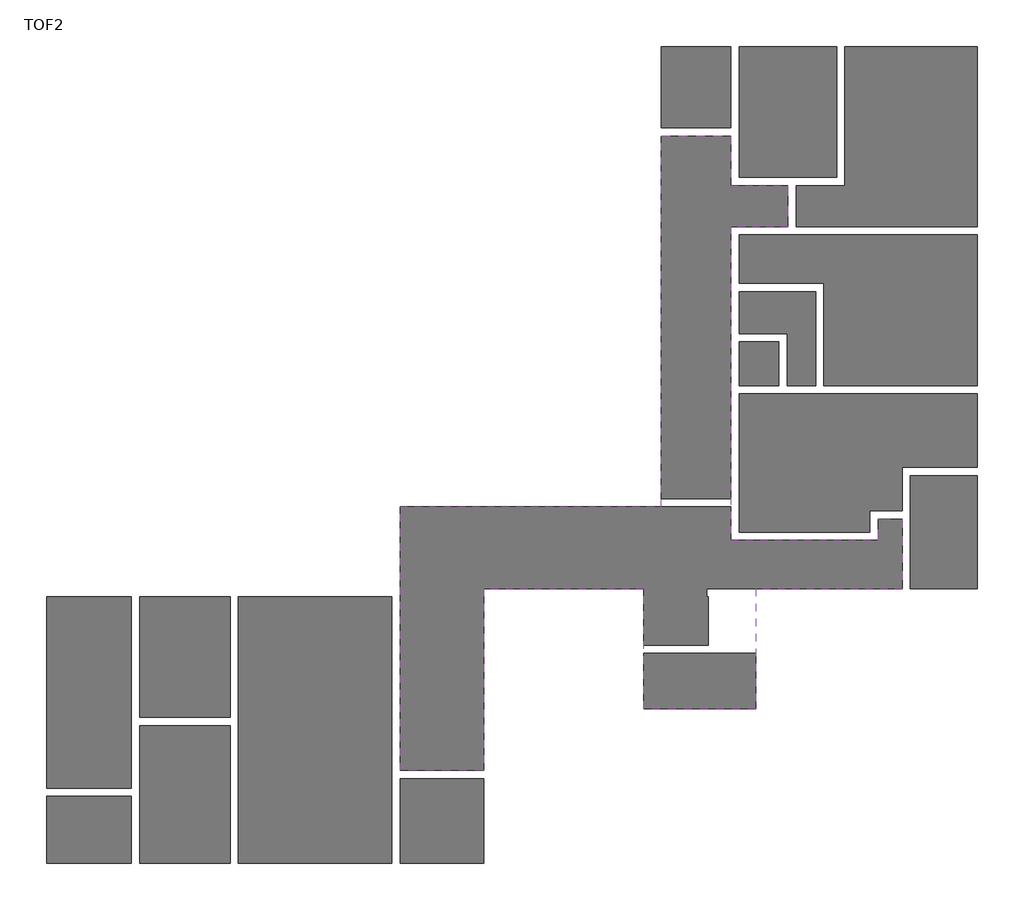
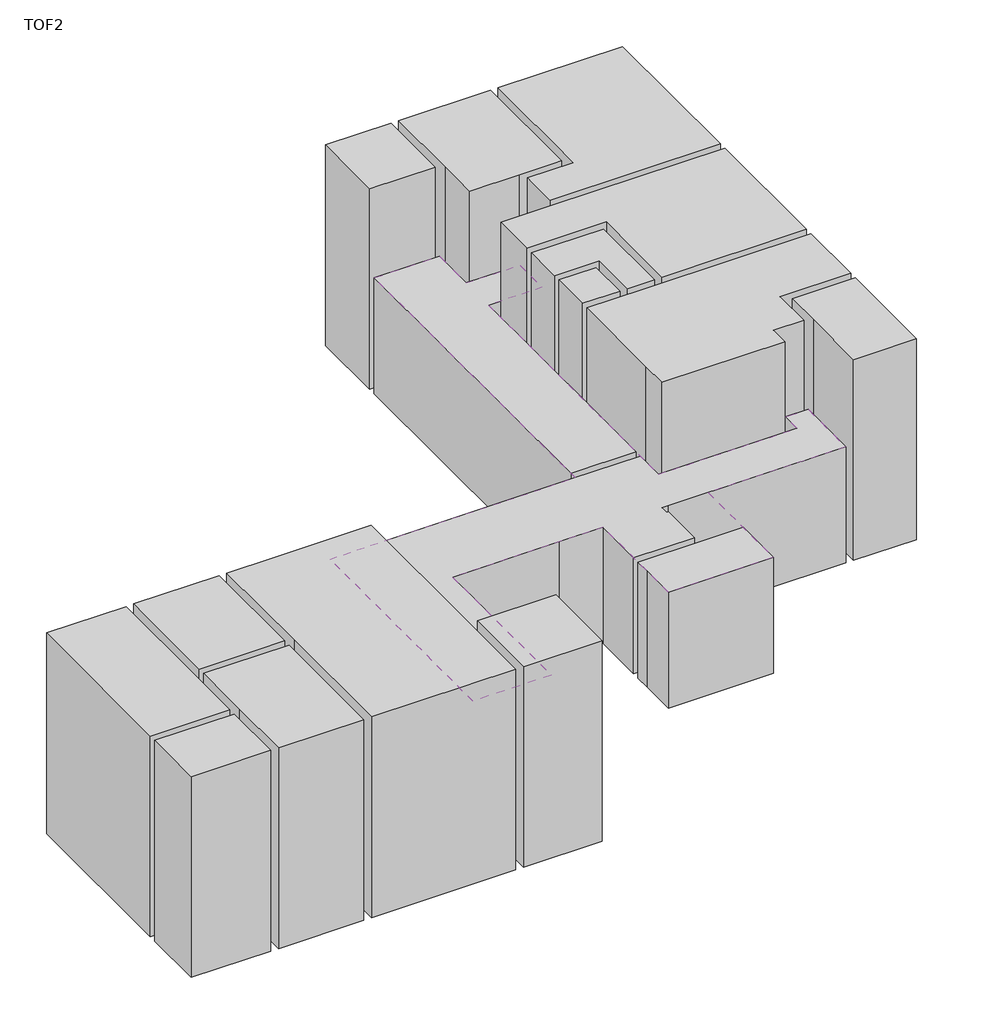
# One storey: 17 proxies, 1 covering.
"""IFC4 building model written with IfcOpenShell, lengths in millimetres."""

from ifc_helpers import new_model, si_unit, frame, origin, place, context, project, spatial, polyline, outline, extrude, element, save

model = new_model("IFC4")

# Units and contexts
model_context = context("Model", 3, world=origin())
ifc_project = project(units=[si_unit("LENGTHUNIT", "METRE", prefix="MILLI")], contexts=[model_context])

# Site, building, storey
site = spatial("IfcSite", under=ifc_project)
building = spatial("IfcBuilding", under=site)
storey = spatial("IfcBuildingStorey", under=building, Name="TOF2", Elevation=1150.0)

# Proxies
placement = place(None, origin())
element("IfcBuildingElementProxy", 1, Name="Generic Models", at=placement, inside=storey, context=model_context, shape_type="SweptSolid", body=[
    extrude(outline(polyline([(29058.7, 8299.5208589), (31624.7, 8299.5208589), (31624.7, 4880.5208589), (29058.7, 4880.5208589), (29058.7, 8299.5208589)])), frame((0.0, 0.0, 1150.0), z_axis=(0.0, 0.0, 1.0), x_axis=(1.0, 0.0, 0.0)), (0.0, 0.0, 1.0), 6399.0),
])
element("IfcBuildingElementProxy", 2, Name="Generic Models", at=placement, inside=storey, context=model_context, shape_type="SweptSolid", body=[
    extrude(outline(polyline([(31624.7, 746.5208589), (29058.7, 746.5208589), (29058.7, 2763.5208589), (29058.7, 4646.5208589), (31624.7, 4646.5208589), (31624.7, 746.5208589)])), frame((0.0, 0.0, 1150.0), z_axis=(0.0, 0.0, 1.0), x_axis=(1.0, 0.0, 0.0)), (0.0, 0.0, 1.0), 6399.0),
])
element("IfcBuildingElementProxy", 3, Name="Generic Models", at=placement, inside=storey, context=model_context, shape_type="SweptSolid", body=[
    extrude(outline(polyline([(26424.7, 8299.5208589), (28824.7, 8299.5208589), (28824.7, 4763.5208589), (28824.7, 2880.5208589), (26424.7, 2880.5208589), (26424.7, 8299.5208589)])), frame((0.0, 0.0, 1150.0), z_axis=(0.0, 0.0, 1.0), x_axis=(1.0, 0.0, 0.0)), (0.0, 0.0, 1.0), 6399.0),
])
element("IfcBuildingElementProxy", 4, Name="Generic Models", at=placement, inside=storey, context=model_context, shape_type="SweptSolid", body=[
    extrude(outline(polyline([(28824.7, 746.5208589), (26424.7, 746.5208589), (26424.7, 2646.5208589), (28824.7, 2646.5208589), (28824.7, 746.5208589)])), frame((0.0, 0.0, 1150.0), z_axis=(0.0, 0.0, 1.0), x_axis=(1.0, 0.0, 0.0)), (0.0, 0.0, 1.0), 6399.0),
])
element("IfcBuildingElementProxy", 5, Name="Generic Models", at=placement, inside=storey, context=model_context, shape_type="SweptSolid", body=[
    extrude(outline(polyline([(52794.7, 14049.5208589), (52794.7, 11967.5208589), (50660.7, 11967.5208589), (50660.7, 10733.5208589), (49743.7, 10733.5208589), (49743.7, 10133.5208589), (46041.7, 10133.5208589), (46041.7, 10966.5208589), (46041.7, 14049.5208589), (46824.7, 14049.5208589), (47924.7, 14049.5208589), (52794.7, 14049.5208589)])), frame((0.0, 0.0, 1150.0), z_axis=(0.0, 0.0, 1.0), x_axis=(1.0, 0.0, 0.0)), (0.0, 0.0, 1.0), 6399.0),
])
element("IfcBuildingElementProxy", 6, Name="Generic Models", at=placement, inside=storey, context=model_context, shape_type="SweptSolid", body=[
    extrude(outline(polyline([(52794.7, 18549.5208589), (52794.7, 14283.5208589), (48441.7, 14283.5208589), (48441.7, 17180.5208589), (46041.7, 17180.5208589), (46041.7, 18549.5208589), (47541.7, 18549.5208589), (52794.7, 18549.5208589)])), frame((0.0, 0.0, 1150.0), z_axis=(0.0, 0.0, 1.0), x_axis=(1.0, 0.0, 0.0)), (0.0, 0.0, 1.0), 6399.0),
])
element("IfcBuildingElementProxy", 7, Name="Generic Models", at=placement, inside=storey, context=model_context, shape_type="SweptSolid", body=[
    extrude(outline(polyline([(46041.7, 15754.2234045), (46041.7, 16946.5208589), (48207.7, 16946.5208589), (48207.7, 14283.5208589), (47401.7, 14283.5208589), (47401.7, 15754.2234045), (46041.7, 15754.2234045)])), frame((0.0, 0.0, 1150.0), z_axis=(0.0, 0.0, 1.0), x_axis=(1.0, 0.0, 0.0)), (0.0, 0.0, 1.0), 6399.0),
])
element("IfcBuildingElementProxy", 8, Name="Generic Models", at=placement, inside=storey, context=model_context, shape_type="SweptSolid", body=[
    extrude(outline(polyline([(46041.7, 14283.5208589), (46041.7, 15520.2234045), (47167.7, 15520.2234045), (47167.7, 14283.5208589), (46041.7, 14283.5208589)])), frame((0.0, 0.0, 1150.0), z_axis=(0.0, 0.0, 1.0), x_axis=(1.0, 0.0, 0.0)), (0.0, 0.0, 1.0), 6399.0),
])
element("IfcBuildingElementProxy", 9, Name="Generic Models", at=placement, inside=storey, context=model_context, shape_type="SweptSolid", body=[
    extrude(outline(polyline([(43841.7, 23886.5208589), (45807.7, 23886.5208589), (45807.7, 21586.5208589), (43841.7, 21586.5208589), (43841.7, 23886.5208589)])), frame((0.0, 0.0, 1150.0), z_axis=(0.0, 0.0, 1.0), x_axis=(1.0, 0.0, 0.0)), (0.0, 0.0, 1.0), 6399.0),
])
element("IfcBuildingElementProxy", 10, Name="Generic Models", at=placement, inside=storey, context=model_context, shape_type="SweptSolid", body=[
    extrude(outline(polyline([(46041.7, 23886.5208589), (48807.7, 23886.5208589), (48807.7, 20183.5208589), (47541.7, 20183.5208589), (46041.7, 20183.5208589), (46041.7, 21469.5208589), (46041.7, 23886.5208589)])), frame((0.0, 0.0, 1150.0), z_axis=(0.0, 0.0, 1.0), x_axis=(1.0, 0.0, 0.0)), (0.0, 0.0, 1.0), 6399.0),
])
element("IfcBuildingElementProxy", 11, Name="Generic Models", at=placement, inside=storey, context=model_context, shape_type="SweptSolid", body=[
    extrude(outline(polyline([(49041.7, 23886.5208589), (52794.7, 23886.5208589), (52794.7, 18783.5208589), (47658.7, 18783.5208589), (47658.7, 19949.5208589), (49041.7, 19949.5208589), (49041.7, 23886.5208589)])), frame((0.0, 0.0, 1150.0), z_axis=(0.0, 0.0, 1.0), x_axis=(1.0, 0.0, 0.0)), (0.0, 0.0, 1.0), 6399.0),
])
element("IfcBuildingElementProxy", 12, Name="Generic Models", at=placement, inside=storey, context=model_context, shape_type="SweptSolid", body=[
    extrude(outline(polyline([(52794.7, 11733.5208589), (52794.7, 8533.5208589), (50894.7, 8533.5208589), (50894.7, 10616.5208589), (50894.7, 11733.5208589), (52794.7, 11733.5208589)])), frame((0.0, 0.0, 1150.0), z_axis=(0.0, 0.0, 1.0), x_axis=(1.0, 0.0, 0.0)), (0.0, 0.0, 1.0), 6399.0),
])
element("IfcBuildingElementProxy", 13, Name="Generic Models", at=placement, inside=storey, context=model_context, shape_type="SweptSolid", body=[
    extrude(outline(polyline([(36207.7, 746.5208589), (31858.7, 746.5208589), (31858.7, 4763.5208589), (31858.7, 8299.5208589), (33274.7, 8299.5208589), (36207.7, 8299.5208589), (36207.7, 3263.5208589), (36207.7, 746.5208589)])), frame((0.0, 0.0, 1150.0), z_axis=(0.0, 0.0, 1.0), x_axis=(1.0, 0.0, 0.0)), (0.0, 0.0, 1.0), 6399.0),
])
element("IfcBuildingElementProxy", 14, Name="Generic Models", at=placement, inside=storey, context=model_context, shape_type="SweptSolid", body=[
    extrude(outline(polyline([(38807.7, 746.5208589), (36441.7, 746.5208589), (36441.7, 3146.5208589), (38807.7, 3146.5208589), (38807.7, 746.5208589)])), frame((0.0, 0.0, 1150.0), z_axis=(0.0, 0.0, 1.0), x_axis=(1.0, 0.0, 0.0)), (0.0, 0.0, 1.0), 6399.0),
])
element("IfcBuildingElementProxy", 15, Name="Generic Models", at=placement, inside=storey, context=model_context, shape_type="SweptSolid", body=[
    extrude(outline(polyline([(36441.7, 3380.5208589), (36441.7, 8416.5208589), (36441.7, 10849.5208589), (43724.7, 10849.5208589), (45807.7, 10849.5208589), (45807.7, 9899.5208589), (49977.7, 9899.5208589), (49977.7, 10499.5208589), (50660.7, 10499.5208589), (50660.7, 8533.5208589), (45292.8778017, 8533.5208589), (45124.7, 8533.5208589), (45124.7, 8299.5208589), (45175.8778017, 8299.5208589), (45175.8778017, 6933.5208589), (43341.7, 6933.5208589), (43341.7, 8533.5208589), (42007.7, 8533.5208589), (38807.7, 8533.5208589), (38807.7, 6963.5208589), (38807.7, 5013.5208589), (38807.7, 3380.5208589), (36441.7, 3380.5208589)])), frame((0.0, 0.0, 1150.0), z_axis=(0.0, 0.0, 1.0), x_axis=(1.0, 0.0, 0.0)), (0.0, 0.0, 1.0), 3700.0),
])
element("IfcBuildingElementProxy", 16, Name="Generic Models", at=placement, inside=storey, context=model_context, shape_type="SweptSolid", body=[
    extrude(outline(polyline([(46507.7, 6699.5208589), (46507.7, 5130.5208589), (43341.7, 5130.5208589), (43341.7, 6216.5208589), (43341.7, 6699.5208589), (45292.8778017, 6699.5208589), (46507.7, 6699.5208589)])), frame((0.0, 0.0, 1150.0), z_axis=(0.0, 0.0, 1.0), x_axis=(1.0, 0.0, 0.0)), (0.0, 0.0, 1.0), 3700.0),
])
element("IfcBuildingElementProxy", 17, Name="Generic Models", at=placement, inside=storey, context=model_context, shape_type="SweptSolid", body=[
    extrude(outline(polyline([(45807.7, 11083.5208589), (43841.7, 11083.5208589), (43841.7, 21352.5208589), (45807.7, 21352.5208589), (45807.7, 19949.5208589), (47424.7, 19949.5208589), (47424.7, 18783.5208589), (45807.7, 18783.5208589), (45807.7, 16283.5208589), (45807.7, 15183.5208589), (45807.7, 14166.5208589), (45807.7, 11083.5208589)])), frame((0.0, 0.0, 1150.0), z_axis=(0.0, 0.0, 1.0), x_axis=(1.0, 0.0, 0.0)), (0.0, 0.0, 1.0), 3700.0),
])

# Covering
element("IfcCovering", 18, ObjectType="CE741_Acoustic Tiled Ceiling System_600x600x9t_T_bar", at=placement, inside=storey, context=model_context, shape_type="SweptSolid", body=[
    extrude(outline(polyline([(46507.7, 8533.5208589), (46507.7, 5130.5208589), (43341.7, 5130.5208589), (43341.7, 8533.5208589), (38807.7, 8533.5208589), (38807.7, 3380.5208589), (36441.7, 3380.5208589), (36441.7, 10849.5208589), (43841.7, 10849.5208589), (43841.7, 21352.5208589), (45807.7, 21352.5208589), (45807.7, 19949.5208589), (47424.7, 19949.5208589), (47424.7, 18783.5208589), (45807.7, 18783.5208589), (45807.7, 9899.5208589), (49977.7, 9899.5208589), (49977.7, 10499.5208589), (50660.7, 10499.5208589), (50660.7, 8533.5208589), (46507.7, 8533.5208589)])), frame((0.0, 0.0, 4850.0), z_axis=(0.0, 0.0, 1.0), x_axis=(1.0, 0.0, 0.0)), (0.0, 0.0, 1.0), 9.0),
])

save(model, "model.ifc")

# Revit data of these elements
# Project information
#   Building Name = "SULFUR LOADING CONTROL BD"
#   Project Status = "Project Status"
#   Client Name = "현대엔지니어링"
#   Project Address = "서울시 종로구 율곡로 75(계동)"
#   Project Number = "-"
# Grids (mm)
#   "Y1": line (-3935.398, 24016.521) -> (58968.688, 24016.521)
#   "X1": line (-75.3, 29394.337) -> (-75.3, -4379.638)
#   "X2": line (5924.7, 29394.337) -> (5924.7, -4379.638)
#   "Y3": line (-3935.398, 8416.521) -> (58968.688, 8416.521)
#   "Y4": line (-3935.398, 616.521) -> (58968.688, 616.521)
#   "X3": line (11924.7, 29394.337) -> (11924.7, -4379.638)
#   "X4": line (17924.7, 29394.337) -> (17924.7, -4379.638)
#   "X5": line (26124.7, 29394.337) -> (26124.7, -4379.638)
#   "X6": line (31924.7, 29394.337) -> (31924.7, -4379.638)
#   "X7": line (38924.7, 29394.337) -> (38924.7, -4379.638)
#   "X8": line (45924.7, 29394.337) -> (45924.7, -4379.638)
#   "X9": line (52924.7, 29394.337) -> (52924.7, -4379.638)
#   "X15": line (43724.7, 27041.858) -> (43724.7, 9156.488)
#   "X16": line (36324.7, 27041.858) -> (36324.7, 9156.488)
#   "X17": line (34685.051, 10966.521) -> (55094.626, 10966.521)
#   "X18": line (34685.051, 18666.521) -> (55094.626, 18666.521)
#   "Y2": line (-3935.398, 12316.521) -> (58968.688, 12316.521)
# Type "CE741_Acoustic Tiled Ceiling System_600x600x9t_T_bar"
#   built-in parameter 1002203 = 1 (stored number, unit not read)
#   built-in parameter 1002202 = 1 (stored number, unit not read)
#   Layers, outside or top first: 9.000 mm no material (function 4)
# Elements 1, 2, 3, 4, 5, 6, 7, 8, 9, 10, 11, 12, 13, 14, 15, 16, 17 (IfcBuildingElementProxy)
#   Phase Created = New Construction
#   Materials on its faces: "Default"
# Element 18 (IfcCovering, "CE741_Acoustic Tiled Ceiling System_600x600x9t_T_bar")
#   Height Offset From Level = 3700.000 mm
#   Phase Created = New Construction
# Materials
#   "Default": class "Miscellaneous", colour RGB 80 80 80, transparency 0
# Room at (42616.2, 7496.521) mm, phase "New Construction", upper level "TOC", upper offset 6500.000 mm, lower offset -1000.000 mm
#   Comments = ""
#   Number = "127"
#   Name = "SHOWER ROOM"
#   Floor Finish Style Name = "Non-Slip Unglazed Ceramic Tile on Screed + Liquid Waterproofing"
#   Floor Finish Ref. = ""
#   Floor-Base Material = "Concrete Slab"
#   Floor Finish-1 = "Screed"
#   Floor Finish-2 = "Liquid Waterproofing"
#   Floor Finish-3 = "Ceramic Tile"
#   Floor Finish-4 = ""
#   Base Finish Style Name = "Epoxy Paint"
#   Base Finish Ref. = ""
#   Base-Base Material = "Concrete Wall\n/ Masonry Wall \n/ Dry Wall"
#   Base Finish-1 = ""
#   Base Finish-2 = ""
#   Base Finish-3 = "Epoxy Paint"
#   Base Finish-4 = ""
#   Wall Finish-1 = "Glazed Ceramic Tile on Cement Plaster"
#   Wall Finish-2 = "No Ceiling\nFull Height"
#   Wall Finish-3 = "Concrete Wall\n/ Masonry Wall"
#   Wall Finish-4 = "Plastering (Tile Workì í¬í¨)"
#   Ceiling Finish Style Name = "Suspended Moisture Resistant Tiled Ceiling (T-Bar)"
#   Ceiling Finish Ref. = "600x600\nT bar"
#   Ceiling-Base Material = "Concrete Slab"
#   Ceiling Finish-1 = ""
#   Ceiling Finish-2 = ""
#   Ceiling Finish-3 = "Moisture Resistant Tiled Ceiling System (T-Bar)"
#   Ceiling Finish-4 = ""
#   H_Room L = 1800.000 mm
#   H_Room W = 1200.000 mm
#   H_Room H or CH = 7300.000 mm
#   Floor Finish Style No = F31B
#   Base Finish Style No = B03
#   Wall Finish Style No = W32C
#   Ceiling Finish Style No = C96A
# Room at (42616.2, 5955.021) mm, phase "New Construction", upper level "TOC", upper offset 6500.000 mm, lower offset -1000.000 mm
#   Comments = ""
#   Number = "128"
#   Name = "EWH ROOM"
#   Floor Finish Style Name = "Non-Slip Unglazed Ceramic Tile on Screed"
#   Floor Finish Ref. = ""
#   Floor-Base Material = "Concrete Slab"
#   Floor Finish-1 = "Screed"
#   Floor Finish-2 = ""
#   Floor Finish-3 = "Ceramic Tile"
#   Floor Finish-4 = ""
#   Base Finish Style Name = "Epoxy Paint"
#   Base Finish Ref. = ""
#   Base-Base Material = "Concrete Wall\n/ Masonry Wall \n/ Dry Wall"
#   Base Finish-1 = ""
#   Base Finish-2 = ""
#   Base Finish-3 = "Epoxy Paint"
#   Base Finish-4 = ""
#   Wall Finish-1 = "Acrylic Emulsion Paint on Cement Plaster"
#   Wall Finish-2 = "T13 Plaster"
#   Wall Finish-3 = "Masonry Wall"
#   Wall Finish-4 = "Plastering"
#   Ceiling Finish Style Name = "Suspended Acoustic Tiled Ceiling (T-Bar)"
#   Ceiling Finish Ref. = "600x600\nT Bar"
#   Ceiling-Base Material = "Concrete Slab"
#   Ceiling Finish-1 = ""
#   Ceiling Finish-2 = ""
#   Ceiling Finish-3 = "Acoustic Tiled Ceiling System (T-Bar)"
#   Ceiling Finish-4 = ""
#   H_Room L = 1500.000 mm
#   H_Room W = 1200.000 mm
#   H_Room H or CH = 7300.000 mm
#   Floor Finish Style No = F31A
#   Base Finish Style No = B03
#   Wall Finish Style No = W01B
#   Ceiling Finish Style No = C95A
# Room at (30341.7, 6590.021) mm, phase "New Construction", upper level "TOC", upper offset 6500.000 mm, lower offset -1000.000 mm
#   Comments = ""
#   Number = "113"
#   Name = "STORE"
#   Floor Finish Style Name = "Vinyl Tile on Screed"
#   Floor Finish Ref. = ""
#   Floor-Base Material = "Concrete Slab"
#   Floor Finish-1 = "Screed"
#   Floor Finish-2 = ""
#   Floor Finish-3 = "Vinyl Tile"
#   Floor Finish-4 = ""
#   Base Finish Style Name = "Coved Vinyl Tile"
#   Base Finish Ref. = ""
#   Base-Base Material = "Concrete Wall\n/ Masonry Wall"
#   Base Finish-1 = ""
#   Base Finish-2 = ""
#   Base Finish-3 = "Vinyl Tile"
#   Base Finish-4 = ""
#   Wall Finish-1 = "Acrylic Emulsion Paint on Cement Plaster"
#   Wall Finish-2 = "T13 Plaster"
#   Wall Finish-3 = "Masonry Wall"
#   Wall Finish-4 = "Plastering"
#   Ceiling Finish Style Name = "Suspended Acoustic Tiled Ceiling (T-Bar)"
#   Ceiling Finish Ref. = "600x600\nT Bar"
#   Ceiling-Base Material = "Concrete Slab"
#   Ceiling Finish-1 = ""
#   Ceiling Finish-2 = ""
#   Ceiling Finish-3 = "Acoustic Tiled Ceiling System (T-Bar)"
#   Ceiling Finish-4 = ""
#   H_Room L = 3600.000 mm
#   H_Room W = 2700.000 mm
#   H_Room H or CH = 6300.000 mm
#   Floor Finish Style No = F34A
#   Base Finish Style No = B35A
#   Wall Finish Style No = W01B
#   Ceiling Finish Style No = C95A
# Room at (30341.7, 2647.521) mm, phase "New Construction", upper level "TOC", upper offset 6500.000 mm, lower offset -1000.000 mm
#   Comments = ""
#   Number = "115"
#   Name = "TELECOMS ROOM"
#   Floor Finish Style Name = "Vinyl Tile on Screed"
#   Floor Finish Ref. = ""
#   Floor-Base Material = "Concrete Slab"
#   Floor Finish-1 = "Screed"
#   Floor Finish-2 = ""
#   Floor Finish-3 = "Vinyl Tile"
#   Floor Finish-4 = ""
#   Base Finish Style Name = "Coved Vinyl Tile"
#   Base Finish Ref. = ""
#   Base-Base Material = "Concrete Wall\n/ Masonry Wall"
#   Base Finish-1 = ""
#   Base Finish-2 = ""
#   Base Finish-3 = "Vinyl Tile"
#   Base Finish-4 = ""
#   Wall Finish-1 = "2 Coats of Non-Conductive & Fire Retardant White Color Paint on Thk.13 Cement Plaster"
#   Wall Finish-2 = ""
#   Wall Finish-3 = ""
#   Wall Finish-4 = ""
#   Ceiling Finish Style Name = "Acrylic Emulsion Paint on Fair Faced Concrete"
#   Ceiling Finish Ref. = ""
#   Ceiling-Base Material = "Concrete Slab"
#   Ceiling Finish-1 = ""
#   Ceiling Finish-2 = ""
#   Ceiling Finish-3 = "Acrylic Emulsion Paint"
#   Ceiling Finish-4 = ""
#   H_Room L = 4200.000 mm
#   H_Room W = 2700.000 mm
#   H_Room H or CH = 6300.000 mm
#   Floor Finish Style No = F34A
#   Base Finish Style No = B35A
#   Wall Finish Style No = W11
#   Ceiling Finish Style No = C01
# Room at (27624.7, 5590.021) mm, phase "New Construction", upper level "TOC", upper offset 6500.000 mm, lower offset -1000.000 mm
#   Comments = ""
#   Number = "116"
#   Name = "CORRIDOR"
#   Floor Finish Style Name = "Vinyl Tile on Screed"
#   Floor Finish Ref. = ""
#   Floor-Base Material = "Concrete Slab"
#   Floor Finish-1 = "Screed"
#   Floor Finish-2 = ""
#   Floor Finish-3 = "Vinyl Tile"
#   Floor Finish-4 = ""
#   Base Finish Style Name = "Coved Vinyl Tile"
#   Base Finish Ref. = ""
#   Base-Base Material = "Concrete Wall\n/ Masonry Wall"
#   Base Finish-1 = ""
#   Base Finish-2 = ""
#   Base Finish-3 = "Vinyl Tile"
#   Base Finish-4 = ""
#   Wall Finish-1 = "Acrylic Emulsion Paint on Cement Plaster"
#   Wall Finish-2 = "T13 Plaster"
#   Wall Finish-3 = "Masonry Wall"
#   Wall Finish-4 = "Plastering"
#   Ceiling Finish Style Name = "Suspended Acoustic Tiled Ceiling (T-Bar)"
#   Ceiling Finish Ref. = "600x600\nT Bar"
#   Ceiling-Base Material = "Concrete Slab"
#   Ceiling Finish-1 = ""
#   Ceiling Finish-2 = ""
#   Ceiling Finish-3 = "Acoustic Tiled Ceiling System (T-Bar)"
#   Ceiling Finish-4 = ""
#   H_Room L = 5600.000 mm
#   H_Room W = 2600.000 mm
#   H_Room H or CH = 6300.000 mm
#   Floor Finish Style No = F34A
#   Base Finish Style No = B35A
#   Wall Finish Style No = W01B
#   Ceiling Finish Style No = C95A
# Room at (27624.7, 1647.521) mm, phase "New Construction", upper level "TOC", upper offset 6500.000 mm, lower offset -1000.000 mm
#   Comments = ""
#   Number = "117"
#   Name = "AIR LOCK"
#   Floor Finish Style Name = "Vinyl Tile on Screed + Matwell"
#   Base Finish Style Name = "Coved Vinyl Tile"
#   Base Finish Ref. = ""
#   Base-Base Material = "Concrete Wall\n/ Masonry Wall"
#   Base Finish-1 = ""
#   Base Finish-2 = ""
#   Base Finish-3 = "Vinyl Tile"
#   Base Finish-4 = ""
#   Wall Finish-1 = "Acrylic Emulsion Paint on Cement Plaster"
#   Wall Finish-2 = "T13 Plaster"
#   Wall Finish-3 = "Masonry Wall"
#   Wall Finish-4 = "Plastering"
#   Ceiling Finish Style Name = "Suspended Acoustic Tiled Ceiling (T-Bar)"
#   Ceiling Finish Ref. = "600x600\nT Bar"
#   Ceiling-Base Material = "Concrete Slab"
#   Ceiling Finish-1 = ""
#   Ceiling Finish-2 = ""
#   Ceiling Finish-3 = "Acoustic Tiled Ceiling System (T-Bar)"
#   Ceiling Finish-4 = ""
#   H_Room L = 2200.000 mm
#   H_Room W = 2600.000 mm
#   H_Room H or CH = 6300.000 mm
#   Floor Finish Style No = F34A-1
#   Base Finish Style No = B35A
#   Wall Finish Style No = W01B
#   Ceiling Finish Style No = C95A
# Room at (49467.2, 12091.521) mm, phase "New Construction", upper level "TOC", upper offset 6500.000 mm, lower offset -1000.000 mm
#   Comments = ""
#   Number = "111"
#   Name = "PRAYER ROOM"
#   Floor Finish Style Name = "Carpet Tile on Screed"
#   Floor Finish Ref. = ""
#   Floor-Base Material = "Concrete Slab"
#   Floor Finish-1 = "Screed"
#   Floor Finish-2 = ""
#   Floor Finish-3 = "Carpet Tile"
#   Floor Finish-4 = ""
#   Base Finish Style Name = "Coved Vinyl Tile"
#   Base Finish Ref. = ""
#   Base-Base Material = "Concrete Wall\n/ Masonry Wall"
#   Base Finish-1 = ""
#   Base Finish-2 = ""
#   Base Finish-3 = "Vinyl Tile"
#   Base Finish-4 = ""
#   Wall Finish-1 = "Acrylic Emulsion Paint on Cement Plaster"
#   Wall Finish-2 = "T13 Plaster"
#   Wall Finish-3 = "Masonry Wall"
#   Wall Finish-4 = "Plastering"
#   Ceiling Finish Style Name = "Suspended Acoustic Tiled Ceiling (T-Bar)"
#   Ceiling Finish Ref. = "600x600\nT Bar"
#   Ceiling-Base Material = "Concrete Slab"
#   Ceiling Finish-1 = ""
#   Ceiling Finish-2 = ""
#   Ceiling Finish-3 = "Acoustic Tiled Ceiling System (T-Bar)"
#   Ceiling Finish-4 = ""
#   H_Room L = 4100.000 mm
#   H_Room W = 7000.000 mm
#   H_Room H or CH = 6300.000 mm
#   Floor Finish Style No = F72
#   Base Finish Style No = B35A
#   Wall Finish Style No = W01B
#   Ceiling Finish Style No = C95A
# Room at (49867.2, 16696.521) mm, phase "New Construction", upper level "TOC", upper offset 6500.000 mm, lower offset -1000.000 mm
#   Comments = ""
#   Number = "108"
#   Name = "BREAK ROOM"
#   Floor Finish Style Name = "Vinyl Tile on Screed"
#   Floor Finish Ref. = ""
#   Floor-Base Material = "Concrete Slab"
#   Floor Finish-1 = "Screed"
#   Floor Finish-2 = ""
#   Floor Finish-3 = "Vinyl Tile"
#   Floor Finish-4 = ""
#   Base Finish Style Name = "Coved Vinyl Tile"
#   Base Finish Ref. = ""
#   Base-Base Material = "Concrete Wall\n/ Masonry Wall"
#   Base Finish-1 = ""
#   Base Finish-2 = ""
#   Base Finish-3 = "Vinyl Tile"
#   Base Finish-4 = ""
#   Wall Finish-1 = "Acrylic Emulsion Paint on Cement Plaster"
#   Wall Finish-2 = "T13 Plaster"
#   Wall Finish-3 = "Masonry Wall"
#   Wall Finish-4 = "Plastering"
#   Ceiling Finish Style Name = "Suspended Moisture Resistant Tiled Ceiling (T-Bar)"
#   Ceiling Finish Ref. = "600x600\nT bar"
#   Ceiling-Base Material = "Concrete Slab"
#   Ceiling Finish-1 = ""
#   Ceiling Finish-2 = ""
#   Ceiling Finish-3 = "Moisture Resistant Tiled Ceiling System (T-Bar)"
#   Ceiling Finish-4 = ""
#   H_Room L = 4500.000 mm
#   H_Room W = 7000.000 mm
#   H_Room H or CH = 6300.000 mm
#   Floor Finish Style No = F34A
#   Base Finish Style No = B35A
#   Wall Finish Style No = W01B
#   Ceiling Finish Style No = C96A
# Room at (47653.075, 16372.8) mm, phase "New Construction", upper level "TOC", upper offset 6500.000 mm, lower offset -1000.000 mm
#   Comments = ""
#   Number = "109"
#   Name = "JANITOR"
#   Floor Finish Style Name = "Non-Slip Unglazed Ceramic Tile on Screed + Liquid Waterproofing"
#   Floor Finish Ref. = ""
#   Floor-Base Material = "Concrete Slab"
#   Floor Finish-1 = "Screed"
#   Floor Finish-2 = "Liquid Waterproofing"
#   Floor Finish-3 = "Ceramic Tile"
#   Floor Finish-4 = ""
#   Base Finish Style Name = "Coved Ceramic Tile"
#   Base Finish Ref. = ""
#   Base-Base Material = "Concrete Wall\n/ Masonry Wall"
#   Base Finish-1 = ""
#   Base Finish-2 = ""
#   Base Finish-3 = "Glazed Ceramic Tile"
#   Base Finish-4 = ""
#   Wall Finish-1 = "Glazed Ceramic Tile (<=2100) / Acrylic Emulsion Paint (>2100) on Cement Plaster"
#   Wall Finish-2 = "H=2100"
#   Ceiling Finish Style Name = "Suspended Moisture Resistant Tiled Ceiling (T-Bar)"
#   Ceiling Finish Ref. = "600x600\nT bar"
#   Ceiling-Base Material = "Concrete Slab"
#   Ceiling Finish-1 = ""
#   Ceiling Finish-2 = ""
#   Ceiling Finish-3 = "Moisture Resistant Tiled Ceiling System (T-Bar)"
#   Ceiling Finish-4 = ""
#   H_Room L = 2800.000 mm
#   H_Room W = 2400.000 mm
#   H_Room H or CH = 6300.000 mm
#   Floor Finish Style No = F31B
#   Base Finish Style No = B32
#   Wall Finish Style No = W32B-1
#   Ceiling Finish Style No = C96A
# Room at (46834.7, 14675.021) mm, phase "New Construction", upper level "TOC", upper offset 6500.000 mm, lower offset -1000.000 mm
#   Comments = ""
#   Number = "126"
#   Name = "EWH ROOM"
#   Floor Finish Style Name = "Vinyl Tile on Screed"
#   Floor Finish Ref. = ""
#   Floor-Base Material = "Concrete Slab"
#   Floor Finish-1 = "Screed"
#   Floor Finish-2 = ""
#   Floor Finish-3 = "Vinyl Tile"
#   Floor Finish-4 = ""
#   Base Finish Style Name = "Coved Vinyl Tile"
#   Base Finish Ref. = ""
#   Base-Base Material = "Concrete Wall\n/ Masonry Wall"
#   Base Finish-1 = ""
#   Base Finish-2 = ""
#   Base Finish-3 = "Vinyl Tile"
#   Base Finish-4 = ""
#   Wall Finish-1 = "Acrylic Emulsion Paint on Cement Plaster"
#   Wall Finish-2 = "T13 Plaster"
#   Wall Finish-3 = "Masonry Wall"
#   Wall Finish-4 = "Plastering"
#   Ceiling Finish Style Name = "Suspended Acoustic Tiled Ceiling (T-Bar)"
#   Ceiling Finish Ref. = "600x600\nT Bar"
#   Ceiling-Base Material = "Concrete Slab"
#   Ceiling Finish-1 = ""
#   Ceiling Finish-2 = ""
#   Ceiling Finish-3 = "Acoustic Tiled Ceiling System (T-Bar)"
#   Ceiling Finish-4 = ""
#   H_Room L = 1400.000 mm
#   H_Room W = 1300.000 mm
#   H_Room H or CH = 6300.000 mm
#   Floor Finish Style No = F34A
#   Base Finish Style No = B35A
#   Wall Finish Style No = W01B
#   Ceiling Finish Style No = C95A
# Room at (8882.2, 18409.021) mm, phase "New Construction", upper level "TOC", upper offset 6500.000 mm, lower offset -1000.000 mm
#   Comments = ""
#   Number = "101"
#   Name = "MECHANICAL ROOM [F-1]"
#   Floor Finish Style Name = "Non-Slip Epoxy Paint on Steel Trowel Finish"
#   Floor Finish Ref. = ""
#   Floor-Base Material = "Concrete Slab"
#   Floor Finish-1 = "Steel Trowel Finish"
#   Floor Finish-2 = ""
#   Floor Finish-3 = "Epoxy Paint"
#   Floor Finish-4 = ""
#   Base Finish Style Name = "Epoxy Paint"
#   Base Finish Ref. = ""
#   Base-Base Material = "Concrete Wall\n/ Masonry Wall \n/ Dry Wall"
#   Base Finish-1 = ""
#   Base Finish-2 = ""
#   Base Finish-3 = "Epoxy Paint"
#   Base Finish-4 = ""
#   Wall Finish-1 = "Acrylic Emulsion Paint on Cement Plaster"
#   Wall Finish-2 = "T13 Plaster"
#   Wall Finish-3 = "Masonry Wall"
#   Wall Finish-4 = "Plastering"
#   Ceiling Finish Style Name = "Acrylic Emulsion Paint on Fair Faced Concrete"
#   Ceiling Finish Ref. = ""
#   Ceiling-Base Material = "Concrete Slab"
#   Ceiling Finish-1 = ""
#   Ceiling Finish-2 = ""
#   Ceiling Finish-3 = "Acrylic Emulsion Paint"
#   Ceiling Finish-4 = ""
#   H_Room L = 11700.000 mm
#   H_Room W = 18000.000 mm
#   H_Room H or CH = 7300.000 mm
#   Floor Finish Style No = F06A
#   Base Finish Style No = B03
#   Wall Finish Style No = W01B
#   Ceiling Finish Style No = C01
# Room at (38499.7, 16059.021) mm, phase "New Construction", upper level "TOC", upper offset 6500.000 mm, lower offset -1000.000 mm
#   Comments = ""
#   Number = "103"
#   Name = "CONTROL ROOM [F-1]"
#   Floor Finish Style Name = "Anti-Dust Epoxy Paint on Steel trowel Finish + Anti-Static Vinyl Tile on Raised Floor"
#   Floor Finish Ref. = "600x600, H=1000"
#   Floor-Base Material = "Concrete Slab"
#   Floor Finish-1 = "Steel Trowel Finish"
#   Floor Finish-2 = "Anti-Dust Paint"
#   Floor Finish-3 = "Raised Floor_Anti-Static Vinyl Tile"
#   Floor Finish-4 = ""
#   Base Finish Style Name = "Coved Vinyl Tile"
#   Base Finish Ref. = ""
#   Base-Base Material = "Concrete Wall\n/ Masonry Wall"
#   Base Finish-1 = ""
#   Base Finish-2 = ""
#   Base Finish-3 = "Vinyl Tile"
#   Base Finish-4 = ""
#   Wall Finish-1 = "Acrylic Emulsion Paint on Cement Plaster"
#   Wall Finish-2 = "T13 Plaster"
#   Wall Finish-3 = "Masonry Wall"
#   Wall Finish-4 = "Plastering"
#   Ceiling Finish Style Name = "Suspended Acoustic Tiled Ceiling (T-Bar)"
#   Ceiling Finish Ref. = "600x600\nT Bar"
#   Ceiling-Base Material = "Concrete Slab"
#   Ceiling Finish-1 = ""
#   Ceiling Finish-2 = ""
#   Ceiling Finish-3 = "Acoustic Tiled Ceiling System (T-Bar)"
#   Ceiling Finish-4 = ""
#   H_Room L = 15600.000 mm
#   H_Room W = 10400.000 mm
#   H_Room H or CH = 7300.000 mm
#   Floor Finish Style No = F91
#   Base Finish Style No = B35A
#   Wall Finish Style No = W01B
#   Ceiling Finish Style No = C95A
# Room at (44824.7, 22985.521) mm, phase "New Construction", upper level "TOC", upper offset 6500.000 mm, lower offset -1000.000 mm
#   Comments = ""
#   Number = "104"
#   Name = "AIR LOCK"
#   Floor Finish Style Name = "Vinyl Tile on Screed + Matwell"
#   Base Finish Style Name = "Coved Vinyl Tile"
#   Base Finish Ref. = ""
#   Base-Base Material = "Concrete Wall\n/ Masonry Wall"
#   Base Finish-1 = ""
#   Base Finish-2 = ""
#   Base Finish-3 = "Vinyl Tile"
#   Base Finish-4 = ""
#   Wall Finish-1 = "Acrylic Emulsion Paint on Cement Plaster"
#   Wall Finish-2 = "T13 Plaster"
#   Wall Finish-3 = "Masonry Wall"
#   Wall Finish-4 = "Plastering"
#   Ceiling Finish Style Name = "Suspended Acoustic Tiled Ceiling (T-Bar)"
#   Ceiling Finish Ref. = "600x600\nT Bar"
#   Ceiling-Base Material = "Concrete Slab"
#   Ceiling Finish-1 = ""
#   Ceiling Finish-2 = ""
#   Ceiling Finish-3 = "Acoustic Tiled Ceiling System (T-Bar)"
#   Ceiling Finish-4 = ""
#   H_Room L = 2600.000 mm
#   H_Room W = 2200.000 mm
#   H_Room H or CH = 6300.000 mm
#   Floor Finish Style No = F34A-1
#   Base Finish Style No = B35A
#   Wall Finish Style No = W01B
#   Ceiling Finish Style No = C95A
# Room at (47424.7, 22284.021) mm, phase "New Construction", upper level "TOC", upper offset 6500.000 mm, lower offset -1000.000 mm
#   Comments = ""
#   Number = "105"
#   Name = "LIBRARY"
#   Floor Finish Style Name = "Vinyl Tile on Screed"
#   Floor Finish Ref. = ""
#   Floor-Base Material = "Concrete Slab"
#   Floor Finish-1 = "Screed"
#   Floor Finish-2 = ""
#   Floor Finish-3 = "Vinyl Tile"
#   Floor Finish-4 = ""
#   Base Finish Style Name = "Coved Vinyl Tile"
#   Base Finish Ref. = ""
#   Base-Base Material = "Concrete Wall\n/ Masonry Wall"
#   Base Finish-1 = ""
#   Base Finish-2 = ""
#   Base Finish-3 = "Vinyl Tile"
#   Base Finish-4 = ""
#   Wall Finish-1 = "Acrylic Emulsion Paint on Cement Plaster"
#   Wall Finish-2 = "T13 Plaster"
#   Wall Finish-3 = "Masonry Wall"
#   Wall Finish-4 = "Plastering"
#   Ceiling Finish Style Name = "Suspended Acoustic Tiled Ceiling (T-Bar)"
#   Ceiling Finish Ref. = "600x600\nT Bar"
#   Ceiling-Base Material = "Concrete Slab"
#   Ceiling Finish-1 = ""
#   Ceiling Finish-2 = ""
#   Ceiling Finish-3 = "Acoustic Tiled Ceiling System (T-Bar)"
#   Ceiling Finish-4 = ""
#   H_Room L = 4000.000 mm
#   H_Room W = 3000.000 mm
#   H_Room H or CH = 6300.000 mm
#   Floor Finish Style No = F34A
#   Base Finish Style No = B35A
#   Wall Finish Style No = W01B
#   Ceiling Finish Style No = C95A
# Room at (50025.7, 21584.021) mm, phase "New Construction", upper level "TOC", upper offset 6500.000 mm, lower offset -1000.000 mm
#   Comments = ""
#   Number = "106"
#   Name = "SHIFT SUPERVISOR/DAY SUPERVISOR"
#   Floor Finish Style Name = "Vinyl Tile on Screed"
#   Floor Finish Ref. = ""
#   Floor-Base Material = "Concrete Slab"
#   Floor Finish-1 = "Screed"
#   Floor Finish-2 = ""
#   Floor Finish-3 = "Vinyl Tile"
#   Floor Finish-4 = ""
#   Base Finish Style Name = "Coved Vinyl Tile"
#   Base Finish Ref. = ""
#   Base-Base Material = "Concrete Wall\n/ Masonry Wall"
#   Base Finish-1 = ""
#   Base Finish-2 = ""
#   Base Finish-3 = "Vinyl Tile"
#   Base Finish-4 = ""
#   Wall Finish-1 = "Acrylic Emulsion Paint on Cement Plaster"
#   Wall Finish-2 = "T13 Plaster"
#   Wall Finish-3 = "Masonry Wall"
#   Wall Finish-4 = "Plastering"
#   Ceiling Finish Style Name = "Suspended Acoustic Tiled Ceiling (T-Bar)"
#   Ceiling Finish Ref. = "600x600\nT Bar"
#   Ceiling-Base Material = "Concrete Slab"
#   Ceiling Finish-1 = ""
#   Ceiling Finish-2 = ""
#   Ceiling Finish-3 = "Acoustic Tiled Ceiling System (T-Bar)"
#   Ceiling Finish-4 = ""
#   H_Room L = 5400.000 mm
#   H_Room W = 5400.000 mm
#   H_Room H or CH = 6300.000 mm
#   Floor Finish Style No = F34A
#   Base Finish Style No = B35A
#   Wall Finish Style No = W01B
#   Ceiling Finish Style No = C95A
# Room at (25599.7, 16059.021) mm, phase "New Construction", upper level "TOC", upper offset 6500.000 mm, lower offset -1000.000 mm
#   Comments = ""
#   Number = "102"
#   Name = "RACK ROOM [F-1]"
#   Floor Finish Style Name = "Anti-Dust Epoxy Paint on Steel trowel Finish + Anti-Static Vinyl Tile on Raised Floor"
#   Floor Finish Ref. = "600x600, H=1000"
#   Floor-Base Material = "Concrete Slab"
#   Floor Finish-1 = "Steel Trowel Finish"
#   Floor Finish-2 = "Anti-Dust Paint"
#   Floor Finish-3 = "Raised Floor_Anti-Static Vinyl Tile"
#   Floor Finish-4 = ""
#   Base Finish Style Name = "Coved Vinyl Tile"
#   Base Finish Ref. = ""
#   Base-Base Material = "Concrete Wall\n/ Masonry Wall"
#   Base Finish-1 = ""
#   Base Finish-2 = ""
#   Base Finish-3 = "Vinyl Tile"
#   Base Finish-4 = ""
#   Wall Finish-1 = "Acrylic Emulsion Paint on Cement Plaster"
#   Wall Finish-2 = "T13 Plaster"
#   Wall Finish-3 = "Masonry Wall"
#   Wall Finish-4 = "Plastering"
#   Ceiling Finish Style Name = "Suspended Acoustic Tiled Ceiling (T-Bar)"
#   Ceiling Finish Ref. = "600x600\nT Bar"
#   Ceiling-Base Material = "Concrete Slab"
#   Ceiling Finish-1 = ""
#   Ceiling Finish-2 = ""
#   Ceiling Finish-3 = "Acoustic Tiled Ceiling System (T-Bar)"
#   Ceiling Finish-4 = ""
#   H_Room L = 15600.000 mm
#   H_Room W = 15300.000 mm
#   H_Room H or CH = 3000.000 mm
#   Floor Finish Style No = F91
#   Base Finish Style No = B35A
#   Wall Finish Style No = W01B
#   Ceiling Finish Style No = C95A
# Room at (40466.2, 6715.021) mm, phase "New Construction", upper level "TOC", upper offset 6500.000 mm, lower offset -1000.000 mm
#   Comments = ""
#   Number = "121"
#   Name = "LOCKER"
#   Floor Finish Style Name = "Non-Slip Unglazed Ceramic Tile on Screed"
#   Floor Finish Ref. = ""
#   Floor-Base Material = "Concrete Slab"
#   Floor Finish-1 = "Screed"
#   Floor Finish-2 = ""
#   Floor Finish-3 = "Ceramic Tile"
#   Floor Finish-4 = ""
#   Base Finish Style Name = "Coved Ceramic Tile"
#   Base Finish Ref. = ""
#   Base-Base Material = "Concrete Wall\n/ Masonry Wall"
#   Base Finish-1 = ""
#   Base Finish-2 = ""
#   Base Finish-3 = "Glazed Ceramic Tile"
#   Base Finish-4 = ""
#   Wall Finish-1 = "Glazed Ceramic Tile (<=2100) / Acrylic Emulsion Paint (>2100) on Cement Plaster"
#   Wall Finish-2 = "H=2100"
#   Ceiling Finish Style Name = "Suspended Moisture Resistant Tiled Ceiling (T-Bar)"
#   Ceiling Finish Ref. = "600x600\nT bar"
#   Ceiling-Base Material = "Concrete Slab"
#   Ceiling Finish-1 = ""
#   Ceiling Finish-2 = ""
#   Ceiling Finish-3 = "Moisture Resistant Tiled Ceiling System (T-Bar)"
#   Ceiling Finish-4 = ""
#   H_Room L = 3400.000 mm
#   H_Room W = 3000.000 mm
#   H_Room H or CH = 7300.000 mm
#   Floor Finish Style No = F31A
#   Base Finish Style No = B32
#   Wall Finish Style No = W32B-1
#   Ceiling Finish Style No = C96A
# Room at (51893.7, 10133.521) mm, phase "New Construction", upper level "TOC", upper offset 6500.000 mm, lower offset -1000.000 mm
#   Comments = ""
#   Number = "110"
#   Name = "ABLUTIONS"
#   Floor Finish Style Name = "Non-Slip Unglazed Ceramic Tile on Screed + Liquid Waterproofing"
#   Floor Finish Ref. = ""
#   Floor-Base Material = "Concrete Slab"
#   Floor Finish-1 = "Screed"
#   Floor Finish-2 = "Liquid Waterproofing"
#   Floor Finish-3 = "Ceramic Tile"
#   Floor Finish-4 = ""
#   Base Finish Style Name = "Coved Ceramic Tile"
#   Base Finish Ref. = ""
#   Base-Base Material = "Concrete Wall\n/ Masonry Wall"
#   Base Finish-1 = ""
#   Base Finish-2 = ""
#   Base Finish-3 = "Glazed Ceramic Tile"
#   Base Finish-4 = ""
#   Wall Finish-1 = "Glazed Ceramic Tile (<=2100) / Acrylic Emulsion Paint (>2100) on Cement Plaster"
#   Wall Finish-2 = "H=2100"
#   Ceiling Finish Style Name = "Suspended Moisture Resistant Tiled Ceiling (T-Bar)"
#   Ceiling Finish Ref. = "600x600\nT bar"
#   Ceiling-Base Material = "Concrete Slab"
#   Ceiling Finish-1 = ""
#   Ceiling Finish-2 = ""
#   Ceiling Finish-3 = "Moisture Resistant Tiled Ceiling System (T-Bar)"
#   Ceiling Finish-4 = ""
#   H_Room L = 3400.000 mm
#   H_Room W = 2200.000 mm
#   H_Room H or CH = 6300.000 mm
#   Floor Finish Style No = F31B
#   Base Finish Style No = B32
#   Wall Finish Style No = W32B-1
#   Ceiling Finish Style No = C96A
# Room at (8882.2, 6424.021) mm, phase "New Construction", upper level "TOC", upper offset 6500.000 mm, lower offset -1000.000 mm
#   Comments = ""
#   Number = "112"
#   Name = "ELECTRICAL ROOM(SS08) [F-1]"
#   Floor Finish Style Name = "Non-Slip Epoxy Paint on Screed"
#   Floor Finish Ref. = ""
#   Floor-Base Material = "Concrete Slab"
#   Floor Finish-1 = "Screed"
#   Floor Finish-2 = ""
#   Floor Finish-3 = "Epoxy Paint"
#   Floor Finish-4 = ""
#   Base Finish Style Name = "Epoxy Paint"
#   Base Finish Ref. = ""
#   Base-Base Material = "Concrete Wall\n/ Masonry Wall \n/ Dry Wall"
#   Base Finish-1 = ""
#   Base Finish-2 = ""
#   Base Finish-3 = "Epoxy Paint"
#   Base Finish-4 = ""
#   Wall Finish-1 = "Acrylic Emulsion Paint on Cement Plaster"
#   Wall Finish-2 = "T13 Plaster"
#   Wall Finish-3 = "Masonry Wall"
#   Wall Finish-4 = "Plastering"
#   Ceiling Finish Style Name = "Acrylic Emulsion Paint on Fair Faced Concrete"
#   Ceiling Finish Ref. = ""
#   Ceiling-Base Material = "Concrete Slab"
#   Ceiling Finish-1 = ""
#   Ceiling Finish-2 = ""
#   Ceiling Finish-3 = "Acrylic Emulsion Paint"
#   Ceiling Finish-4 = ""
#   H_Room L = 11700.000 mm
#   H_Room W = 18000.000 mm
#   H_Room H or CH = 7300.000 mm
#   Floor Finish Style No = F06B
#   Base Finish Style No = B03
#   Wall Finish Style No = W01B
#   Ceiling Finish Style No = C01
# Room at (22116.2, 4474.021) mm, phase "New Construction", upper level "TOC", upper offset 6500.000 mm, lower offset -1000.000 mm
#   Comments = ""
#   Number = "114"
#   Name = "BATTERY ROOM [F-1]"
#   Floor Finish Style Name = "Acid Resistant Ceramic Tile on Screed"
#   Floor Finish Ref. = ""
#   Floor-Base Material = "Concrete Slab"
#   Floor Finish-1 = "Screed"
#   Floor Finish-2 = ""
#   Floor Finish-3 = "Acid/Alkaline Resistant Tile"
#   Floor Finish-4 = ""
#   Base Finish Style Name = "Acid Resistant Ceramic Tile"
#   Base Finish Ref. = ""
#   Base-Base Material = "Concrete Wall\n/ Masonry Wall"
#   Base Finish-1 = ""
#   Base Finish-2 = ""
#   Base Finish-3 = "Acid/Alkaline Resistant Tile"
#   Base Finish-4 = ""
#   Wall Finish-1 = "Acid Resistant Paint on Cement Plaster"
#   Wall Finish-2 = "T13 Plaster"
#   Wall Finish-3 = "Masonry Wall"
#   Wall Finish-4 = "Plastering"
#   Ceiling Finish Style Name = "Acrylic Emulsion Paint on Fair Faced Concrete"
#   Ceiling Finish Ref. = ""
#   Ceiling-Base Material = "Concrete Slab"
#   Ceiling Finish-1 = ""
#   Ceiling Finish-2 = ""
#   Ceiling Finish-3 = "Acrylic Emulsion Paint"
#   Ceiling Finish-4 = ""
#   H_Room L = 7800.000 mm
#   H_Room W = 8300.000 mm
#   H_Room H or CH = 7300.000 mm
#   Floor Finish Style No = F32
#   Base Finish Style No = B33
#   Wall Finish Style No = W04B
#   Ceiling Finish Style No = C01
# Room at (34033.2, 4474.021) mm, phase "New Construction", upper level "TOC", upper offset 6500.000 mm, lower offset -1000.000 mm
#   Comments = ""
#   Number = "118"
#   Name = "DRIVERS LOUNGE"
#   Floor Finish Style Name = "Vinyl Tile on Screed"
#   Floor Finish Ref. = ""
#   Floor-Base Material = "Concrete Slab"
#   Floor Finish-1 = "Screed"
#   Floor Finish-2 = ""
#   Floor Finish-3 = "Vinyl Tile"
#   Floor Finish-4 = ""
#   Base Finish Style Name = "Coved Vinyl Tile"
#   Base Finish Ref. = ""
#   Base-Base Material = "Concrete Wall\n/ Masonry Wall"
#   Base Finish-1 = ""
#   Base Finish-2 = ""
#   Base Finish-3 = "Vinyl Tile"
#   Base Finish-4 = ""
#   Wall Finish-1 = "Acrylic Emulsion Paint on Cement Plaster"
#   Wall Finish-2 = "T13 Plaster"
#   Wall Finish-3 = "Masonry Wall"
#   Wall Finish-4 = "Plastering"
#   Ceiling Finish Style Name = "Suspended Acoustic Tiled Ceiling (T-Bar)"
#   Ceiling Finish Ref. = "600x600\nT Bar"
#   Ceiling-Base Material = "Concrete Slab"
#   Ceiling Finish-1 = ""
#   Ceiling Finish-2 = ""
#   Ceiling Finish-3 = "Acoustic Tiled Ceiling System (T-Bar)"
#   Ceiling Finish-4 = ""
#   H_Room L = 7800.000 mm
#   H_Room W = 4500.000 mm
#   H_Room H or CH = 6300.000 mm
#   Floor Finish Style No = F34A
#   Base Finish Style No = B35A
#   Wall Finish Style No = W01B
#   Ceiling Finish Style No = C95A
# Room at (41074.7, 2772.521) mm, phase "New Construction", upper level "TOC", upper offset 6500.000 mm, lower offset -1000.000 mm
#   Comments = ""
#   Number = "122"
#   Name = "TOILETS"
#   Floor Finish Style Name = "Non-Slip Unglazed Ceramic Tile on Screed + Liquid Waterproofing"
#   Floor Finish Ref. = ""
#   Floor-Base Material = "Concrete Slab"
#   Floor Finish-1 = "Screed"
#   Floor Finish-2 = "Liquid Waterproofing"
#   Floor Finish-3 = "Ceramic Tile"
#   Floor Finish-4 = ""
#   Base Finish Style Name = "Coved Ceramic Tile"
#   Base Finish Ref. = ""
#   Base-Base Material = "Concrete Wall\n/ Masonry Wall"
#   Base Finish-1 = ""
#   Base Finish-2 = ""
#   Base Finish-3 = "Glazed Ceramic Tile"
#   Base Finish-4 = ""
#   Wall Finish-1 = "Glazed Ceramic Tile (<=2100) / Acrylic Emulsion Paint (>2100) on Cement Plaster"
#   Wall Finish-2 = "H=2100"
#   Ceiling Finish Style Name = "Suspended Moisture Resistant Tiled Ceiling (T-Bar)"
#   Ceiling Finish Ref. = "600x600\nT bar"
#   Ceiling-Base Material = "Concrete Slab"
#   Ceiling Finish-1 = ""
#   Ceiling Finish-2 = ""
#   Ceiling Finish-3 = "Moisture Resistant Tiled Ceiling System (T-Bar)"
#   Ceiling Finish-4 = ""
#   H_Room L = 4400.000 mm
#   H_Room W = 4300.000 mm
#   H_Room H or CH = 7300.000 mm
#   Floor Finish Style No = F31B
#   Base Finish Style No = B32
#   Wall Finish Style No = W32B-1
#   Ceiling Finish Style No = C96A
# Room at (37624.7, 1897.521) mm, phase "New Construction", upper level "TOC", upper offset 6500.000 mm, lower offset -1000.000 mm
#   Comments = ""
#   Number = "119"
#   Name = "AIR LOCK"
#   Floor Finish Style Name = "Vinyl Tile on Screed + Matwell"
#   Base Finish Style Name = "Coved Vinyl Tile"
#   Base Finish Ref. = ""
#   Base-Base Material = "Concrete Wall\n/ Masonry Wall"
#   Base Finish-1 = ""
#   Base Finish-2 = ""
#   Base Finish-3 = "Vinyl Tile"
#   Base Finish-4 = ""
#   Wall Finish-1 = "Acrylic Emulsion Paint on Cement Plaster"
#   Wall Finish-2 = "T13 Plaster"
#   Wall Finish-3 = "Masonry Wall"
#   Wall Finish-4 = "Plastering"
#   Ceiling Finish Style Name = "Suspended Acoustic Tiled Ceiling (T-Bar)"
#   Ceiling Finish Ref. = "600x600\nT Bar"
#   Ceiling-Base Material = "Concrete Slab"
#   Ceiling Finish-1 = ""
#   Ceiling Finish-2 = ""
#   Ceiling Finish-3 = "Acoustic Tiled Ceiling System (T-Bar)"
#   Ceiling Finish-4 = ""
#   H_Room L = 2700.000 mm
#   H_Room W = 2600.000 mm
#   H_Room H or CH = 6300.000 mm
#   Floor Finish Style No = F34A-1
#   Base Finish Style No = B35A
#   Wall Finish Style No = W01B
#   Ceiling Finish Style No = C95A
# Room at (44924.7, 2772.521) mm, phase "New Construction", upper level "TOC", upper offset 6500.000 mm, lower offset -1000.000 mm
#   Comments = ""
#   Number = "124"
#   Name = "STORE"
#   Floor Finish Style Name = "Vinyl Tile on Screed"
#   Floor Finish Ref. = ""
#   Floor-Base Material = "Concrete Slab"
#   Floor Finish-1 = "Screed"
#   Floor Finish-2 = ""
#   Floor Finish-3 = "Vinyl Tile"
#   Floor Finish-4 = ""
#   Base Finish Style Name = "Coved Vinyl Tile"
#   Base Finish Ref. = ""
#   Base-Base Material = "Concrete Wall\n/ Masonry Wall"
#   Base Finish-1 = ""
#   Base Finish-2 = ""
#   Base Finish-3 = "Vinyl Tile"
#   Base Finish-4 = ""
#   Wall Finish-1 = "Acrylic Emulsion Paint on Cement Plaster"
#   Wall Finish-2 = "T13 Plaster"
#   Wall Finish-3 = "Masonry Wall"
#   Wall Finish-4 = "Plastering"
#   Ceiling Finish Style Name = "Suspended Acoustic Tiled Ceiling (T-Bar)"
#   Ceiling Finish Ref. = "600x600\nT Bar"
#   Ceiling-Base Material = "Concrete Slab"
#   Ceiling Finish-1 = ""
#   Ceiling Finish-2 = ""
#   Ceiling Finish-3 = "Acoustic Tiled Ceiling System (T-Bar)"
#   Ceiling Finish-4 = ""
#   H_Room L = 4400.000 mm
#   H_Room W = 3400.000 mm
#   H_Room H or CH = 7300.000 mm
#   Floor Finish Style No = F34A
#   Base Finish Style No = B35A
#   Wall Finish Style No = W01B
#   Ceiling Finish Style No = C95A
# Room at (49817.2, 4474.021) mm, phase "New Construction", upper level "TOC", upper offset 6500.000 mm, lower offset -1000.000 mm
#   Comments = ""
#   Number = "125"
#   Name = "MAINTENANCE WORKSHOP [F-1]"
#   Floor Finish Style Name = "Non-Slip Epoxy Paint on Steel Trowel Finish"
#   Floor Finish Ref. = ""
#   Floor-Base Material = "Concrete Slab"
#   Floor Finish-1 = "Steel Trowel Finish"
#   Floor Finish-2 = ""
#   Floor Finish-3 = "Epoxy Paint"
#   Floor Finish-4 = ""
#   Base Finish Style Name = "Epoxy Paint"
#   Base Finish Ref. = ""
#   Base-Base Material = "Concrete Wall\n/ Masonry Wall \n/ Dry Wall"
#   Base Finish-1 = ""
#   Base Finish-2 = ""
#   Base Finish-3 = "Epoxy Paint"
#   Base Finish-4 = ""
#   Wall Finish-1 = "Acrylic Emulsion Paint on Cement Plaster"
#   Wall Finish-2 = "T13 Plaster"
#   Wall Finish-3 = "Masonry Wall"
#   Wall Finish-4 = "Plastering"
#   Ceiling Finish Style Name = "Acrylic Emulsion Paint on Fair Faced Concrete"
#   Ceiling Finish Ref. = ""
#   Ceiling-Base Material = "Concrete Slab"
#   Ceiling Finish-1 = ""
#   Ceiling Finish-2 = ""
#   Ceiling Finish-3 = "Acrylic Emulsion Paint"
#   Ceiling Finish-4 = ""
#   H_Room L = 7800.000 mm
#   H_Room W = 7700.000 mm
#   H_Room H or CH = 7300.000 mm
#   Floor Finish Style No = F06A
#   Base Finish Style No = B03
#   Wall Finish Style No = W01B
#   Ceiling Finish Style No = C01
# Room at (43973.125, 9512.388) mm, phase "New Construction", upper level "TOC", upper offset 6500.000 mm, lower offset -1000.000 mm
#   Comments = ""
#   Number = "120"
#   Name = "CORRIDOR"
#   Floor Finish Style Name = "Vinyl Tile on Screed"
#   Floor Finish Ref. = ""
#   Floor-Base Material = "Concrete Slab"
#   Floor Finish-1 = "Screed"
#   Floor Finish-2 = ""
#   Floor Finish-3 = "Vinyl Tile"
#   Floor Finish-4 = ""
#   Base Finish Style Name = "Coved Vinyl Tile"
#   Base Finish Ref. = ""
#   Base-Base Material = "Concrete Wall\n/ Masonry Wall"
#   Base Finish-1 = ""
#   Base Finish-2 = ""
#   Base Finish-3 = "Vinyl Tile"
#   Base Finish-4 = ""
#   Wall Finish-1 = "Acrylic Emulsion Paint on Cement Plaster"
#   Wall Finish-2 = "T13 Plaster"
#   Wall Finish-3 = "Masonry Wall"
#   Wall Finish-4 = "Plastering"
#   Ceiling Finish Style Name = "Suspended Acoustic Tiled Ceiling (T-Bar)"
#   Ceiling Finish Ref. = "600x600\nT Bar"
#   Ceiling-Base Material = "Concrete Slab"
#   Ceiling Finish-1 = ""
#   Ceiling Finish-2 = ""
#   Ceiling Finish-3 = "Acoustic Tiled Ceiling System (T-Bar)"
#   Ceiling Finish-4 = ""
#   H_Room L = 7700.000 mm
#   H_Room W = 14400.000 mm
#   H_Room H or CH = 3600.000 mm
#   Floor Finish Style No = F34A
#   Base Finish Style No = B35A
#   Wall Finish Style No = W01B
#   Ceiling Finish Style No = C95A
# Room at (44840.524, 5924.958) mm, phase "New Construction", upper level "TOC", upper offset 6500.000 mm, lower offset 0.000 mm
#   Comments = ""
#   Number = "123"
#   Name = "STORE"
#   Floor Finish Style Name = "Vinyl Tile on Screed"
#   Floor Finish Ref. = ""
#   Floor-Base Material = "Concrete Slab"
#   Floor Finish-1 = "Screed"
#   Floor Finish-2 = ""
#   Floor Finish-3 = "Vinyl Tile"
#   Floor Finish-4 = ""
#   Base Finish Style Name = "Coved Vinyl Tile"
#   Base Finish Ref. = ""
#   Base-Base Material = "Concrete Wall\n/ Masonry Wall"
#   Base Finish-1 = ""
#   Base Finish-2 = ""
#   Base Finish-3 = "Vinyl Tile"
#   Base Finish-4 = ""
#   Wall Finish-1 = "Acrylic Emulsion Paint on Cement Plaster"
#   Wall Finish-2 = "T13 Plaster"
#   Wall Finish-3 = "Masonry Wall"
#   Wall Finish-4 = "Plastering"
#   Ceiling Finish Style Name = "Suspended Acoustic Tiled Ceiling (T-Bar)"
#   Ceiling Finish Ref. = "600x600\nT Bar"
#   Ceiling-Base Material = "Concrete Slab"
#   Ceiling Finish-1 = ""
#   Ceiling Finish-2 = ""
#   Ceiling Finish-3 = "Acoustic Tiled Ceiling System (T-Bar)"
#   Ceiling Finish-4 = ""
#   H_Room L = 1800.000 mm
#   H_Room W = 3400.000 mm
#   H_Room H or CH = 3700.000 mm
#   Floor Finish Style No = F34A
#   Base Finish Style No = B35A
#   Wall Finish Style No = W01B
#   Ceiling Finish Style No = C95A
# Room at (45068.625, 15370.439) mm, phase "New Construction", upper level "TOC", upper offset 6500.000 mm, lower offset 0.000 mm
#   Comments = ""
#   Number = "107"
#   Name = "CORRIDOR"
#   Floor Finish Style Name = "Vinyl Tile on Screed"
#   Floor Finish Ref. = ""
#   Floor-Base Material = "Concrete Slab"
#   Floor Finish-1 = "Screed"
#   Floor Finish-2 = ""
#   Floor Finish-3 = "Vinyl Tile"
#   Floor Finish-4 = ""
#   Base Finish Style Name = "Coved Vinyl Tile"
#   Base Finish Ref. = ""
#   Base-Base Material = "Concrete Wall\n/ Masonry Wall"
#   Base Finish-1 = ""
#   Base Finish-2 = ""
#   Base Finish-3 = "Vinyl Tile"
#   Base Finish-4 = ""
#   Wall Finish-1 = "Acrylic Emulsion Paint on Cement Plaster"
#   Wall Finish-2 = "T13 Plaster"
#   Wall Finish-3 = "Masonry Wall"
#   Wall Finish-4 = "Plastering"
#   Ceiling Finish Style Name = "Suspended Acoustic Tiled Ceiling (T-Bar)"
#   Ceiling Finish Ref. = "600x600\nT Bar"
#   Ceiling-Base Material = "Concrete Slab"
#   Ceiling Finish-1 = ""
#   Ceiling Finish-2 = ""
#   Ceiling Finish-3 = "Acoustic Tiled Ceiling System (T-Bar)"
#   Ceiling Finish-4 = ""
#   H_Room L = 10500.000 mm
#   H_Room W = 3800.000 mm
#   H_Room H or CH = 3700.000 mm
#   Floor Finish Style No = F34A
#   Base Finish Style No = B35A
#   Wall Finish Style No = W01B
#   Ceiling Finish Style No = C95A
